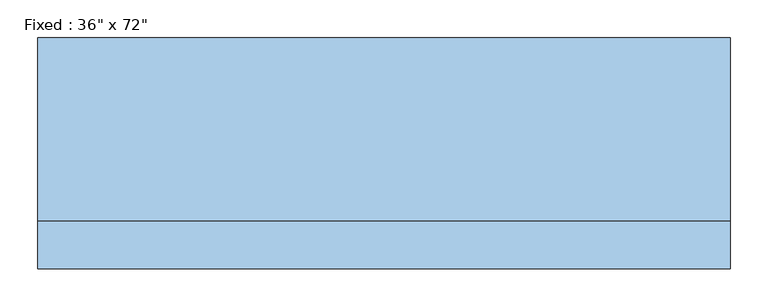
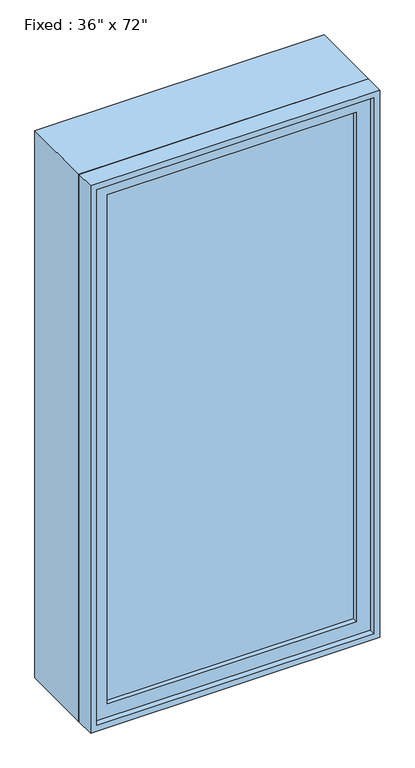
"""IFC4 building model written with IfcOpenShell, lengths in millimetres: window geometry."""

import ifcopenshell
import ifcopenshell.guid

model = None  # the IFC model being written
_history = None  # IfcOwnerHistory: only IFC2X3 demands one
_inside = {}  # id of a spatial element -> (the spatial element, [elements in it])
_under = {}  # id of a project, library or spatial element -> (it, [spatial elements below it])
_declared = {}  # id of a project -> (the project, [libraries it declares])
_typed = {}  # id of a type object -> (the type object, [elements of that type])
_made_of = {}  # id of a material, layer set ... -> (it, [elements and type objects made of it])


def new_model(schema):
    """Start an empty IFC model of exactly this schema.

    Asked for "IFC4X3", IfcOpenShell would pick the latest addendum, in which some entities
    have other attributes; the version numbers below select the first issue.
    IFC2X3 requires an IfcOwnerHistory on every rooted entity: one is made here for all.
    """
    global model, _history
    if schema == "IFC4X3":
        model = ifcopenshell.file(schema_version=(4, 3, 0, 0))
    else:
        model = ifcopenshell.file(schema=schema)
    _inside.clear()
    _under.clear()
    _declared.clear()
    _typed.clear()
    _made_of.clear()
    _history = None
    if model.schema == "IFC2X3":
        org = make("IfcOrganization", Name="unknown")
        user = make(
            "IfcPersonAndOrganization",
            ThePerson=make("IfcPerson", FamilyName="unknown"),
            TheOrganization=org,
        )
        app = make(
            "IfcApplication",
            ApplicationDeveloper=org,
            Version="unknown",
            ApplicationFullName="unknown",
            ApplicationIdentifier="unknown",
        )
        _history = make(
            "IfcOwnerHistory",
            OwningUser=user,
            OwningApplication=app,
            ChangeAction="ADDED",
            CreationDate=0,
        )
    return model


def make(cls, **values):
    """One entity of the class cls with the attributes given. An attribute that is None is left unset."""
    return model.create_entity(
        cls, **{name: value for name, value in values.items() if value is not None}
    )


def rooted(cls, **values):
    """An entity with a GlobalId (a new one), such as an element, a storey or a relation."""
    return make(cls, GlobalId=ifcopenshell.guid.new(), OwnerHistory=_history, **values)


def si_unit(unit_type, name, prefix=None):
    """IfcSIUnit, for example si_unit("LENGTHUNIT", "METRE", prefix="MILLI")."""
    return make("IfcSIUnit", UnitType=unit_type, Prefix=prefix, Name=name)


def assignment(units):
    """IfcUnitAssignment: the units of a project."""
    return None if units is None else make("IfcUnitAssignment", Units=units)


def point(xyz):
    """IfcCartesianPoint."""
    return None if xyz is None else make("IfcCartesianPoint", Coordinates=xyz)


def direction(xyz):
    """IfcDirection."""
    return None if xyz is None else make("IfcDirection", DirectionRatios=xyz)


def frame(location, z_axis=None, x_axis=None):
    """IfcAxis2Placement3D, a coordinate frame: its origin and axes. An axis left out is left unset."""
    return make(
        "IfcAxis2Placement3D",
        Location=point(location),
        Axis=direction(z_axis),
        RefDirection=direction(x_axis),
    )


def origin():
    """The frame at (0, 0, 0) with its axes left unset."""
    return frame((0.0, 0.0, 0.0))


def place(relative_to, where):
    """IfcLocalPlacement: puts the frame where relative to a parent placement (None: the world)."""
    return make(
        "IfcLocalPlacement", PlacementRelTo=relative_to, RelativePlacement=where
    )


def context(
    kind, dimensions, precision=None, world=None, true_north=None, identifier=None
):
    """IfcGeometricRepresentationContext, for example the 3D "Model" context."""
    return make(
        "IfcGeometricRepresentationContext",
        ContextIdentifier=identifier,
        ContextType=kind,
        CoordinateSpaceDimension=dimensions,
        Precision=precision,
        WorldCoordinateSystem=world,
        TrueNorth=true_north,
    )


def project(units=None, contexts=None):
    """IfcProject with its units and contexts."""
    return rooted(
        "IfcProject",
        Name="project",
        RepresentationContexts=contexts,
        UnitsInContext=assignment(units),
    )


def spatial(cls, under=None, at=None, **own):
    """A site, building, storey or space (cls), placed at a placement, below another one or the project."""
    s = rooted(cls, ObjectPlacement=at, **own)
    if under is not None:
        _under.setdefault(under.id(), (under, []))[1].append(s)
    return s


def polyline(points):
    """IfcPolyline through the points."""
    return make("IfcPolyline", Points=[point(p) for p in points])


def outline(outer, holes=None, kind="AREA"):
    """IfcArbitraryClosedProfileDef: a profile drawn as a closed curve; with holes, ...WithVoids."""
    if holes is None:
        return make("IfcArbitraryClosedProfileDef", ProfileType=kind, OuterCurve=outer)
    return make(
        "IfcArbitraryProfileDefWithVoids",
        ProfileType=kind,
        OuterCurve=outer,
        InnerCurves=holes,
    )


def extrude(swept, where, along, depth):
    """IfcExtrudedAreaSolid: the profile swept, set in the frame where, extruded along a direction by depth."""
    return make(
        "IfcExtrudedAreaSolid",
        SweptArea=swept,
        Position=where,
        ExtrudedDirection=direction(along),
        Depth=depth,
    )


def shape(context_of_items, identifier, shape_type, items):
    """IfcShapeRepresentation: the items that make up one representation, for example the "Body"."""
    return make(
        "IfcShapeRepresentation",
        ContextOfItems=context_of_items,
        RepresentationIdentifier=identifier,
        RepresentationType=shape_type,
        Items=items,
    )


def source(mapping_origin, context_of_items, identifier, shape_type, items):
    """IfcRepresentationMap: a shape defined once, which mapped items show again and again."""
    return make(
        "IfcRepresentationMap",
        MappingOrigin=mapping_origin,
        MappedRepresentation=shape(context_of_items, identifier, shape_type, items),
    )


def transform(
    local_origin,
    x_axis=None,
    y_axis=None,
    z_axis=None,
    scale=None,
    scale2=None,
    scale3=None,
    uniform=True,
):
    """IfcCartesianTransformationOperator3D, or its non-uniform kind. x_axis, y_axis, z_axis: its Axis1, 2, 3."""
    if uniform:
        return make(
            "IfcCartesianTransformationOperator3D",
            Axis1=direction(x_axis),
            Axis2=direction(y_axis),
            LocalOrigin=point(local_origin),
            Scale=scale,
            Axis3=direction(z_axis),
        )
    return make(
        "IfcCartesianTransformationOperator3DnonUniform",
        Axis1=direction(x_axis),
        Axis2=direction(y_axis),
        LocalOrigin=point(local_origin),
        Scale=scale,
        Axis3=direction(z_axis),
        Scale2=scale2,
        Scale3=scale3,
    )


def mapped(mapping_source, mapping_target):
    """IfcMappedItem: shows the shape of a source again, moved by a transform."""
    return make(
        "IfcMappedItem", MappingSource=mapping_source, MappingTarget=mapping_target
    )


def made_of(thing, what):
    """Note that an element or type object is made of a material, layer set ...; save() writes the relation."""
    if what is not None:
        _made_of.setdefault(what.id(), (what, []))[1].append(thing)
    return thing


def element(
    cls,
    number,
    at=None,
    inside=None,
    cuts=None,
    type_object=None,
    material=None,
    context=None,
    identifier="Body",
    shape_type=None,
    held_by="IfcProductDefinitionShape",
    body=None,
    shapes=None,
    **own,
):
    """One element of the class cls, such as IfcWall. Its Tag is "e" and its number.

    at: its placement. inside: the storey or other place that contains it. cuts: it is an
    opening in that element (IfcRelVoidsElement). A single representation is given by context,
    identifier, shape_type and body (its items); several are given by shapes. held_by: the class
    of the entity that holds the representations. save() writes the other relations.
    """
    e = rooted(cls, Tag="e%d" % number, ObjectPlacement=at, **own)
    if body is not None:
        shapes = [shape(context, identifier, shape_type, body)]
    if shapes is not None:
        e.Representation = make(held_by, Representations=shapes)
    if inside is not None:
        _inside.setdefault(inside.id(), (inside, []))[1].append(e)
    if cuts is not None:
        rooted(
            "IfcRelVoidsElement", RelatingBuildingElement=cuts, RelatedOpeningElement=e
        )
    if type_object is not None:
        _typed.setdefault(type_object.id(), (type_object, []))[1].append(e)
    return made_of(e, material)


def aggregate(whole, parts):
    """IfcRelAggregates: a whole, such as a stair, and the parts it consists of."""
    return rooted("IfcRelAggregates", RelatingObject=whole, RelatedObjects=parts)


def save(model, path):
    """Write the relations noted so far, then the file.

    IfcRelAggregates (storeys below a building ...), IfcRelContainedInSpatialStructure (elements
    in a storey), IfcRelDefinesByType, IfcRelAssociatesMaterial and IfcRelDeclares: one each for
    every whole, place, type object, material and project.
    """
    for whole, parts in _under.values():
        aggregate(whole, parts)
    for where, things in _inside.values():
        rooted(
            "IfcRelContainedInSpatialStructure",
            RelatedElements=things,
            RelatingStructure=where,
        )
    for kind, things in _typed.values():
        rooted("IfcRelDefinesByType", RelatedObjects=things, RelatingType=kind)
    for what, things in _made_of.values():
        rooted("IfcRelAssociatesMaterial", RelatedObjects=things, RelatingMaterial=what)
    for by, libraries in _declared.values():
        rooted("IfcRelDeclares", RelatingContext=by, RelatedDefinitions=libraries)
    model.write(path)


def window_9a1f8bc2(model_context):
    return source(origin(), model_context, "Body", "SweptSolid", [
        extrude(outline(polyline([(355.6, -104.775), (355.6, -117.475), (-431.8, -117.475), (-431.8, -104.775), (355.6, -104.775)])), frame((0.0, 0.0, 368.3), z_axis=(0.0, 0.0, 1.0), x_axis=(1.0, 0.0, 0.0)), (0.0, 0.0, 1.0), 1701.8),
        extrude(outline(polyline([(2114.55, -476.25), (323.85, -476.25), (323.85, 400.05), (2114.55, 400.05), (2114.55, -476.25)]), holes=[polyline([(2070.1, -431.8), (2070.1, 355.6), (368.3, 355.6), (368.3, -431.8), (2070.1, -431.8)])]), frame((0.0, -133.35, 0.0), z_axis=(0.0, 1.0, 0.0), x_axis=(0.0, 0.0, 1.0)), (0.0, 0.0, 1.0), 44.45),
        extrude(outline(polyline([(2133.6, -495.3), (304.8, -495.3), (304.8, 419.1), (2133.6, 419.1), (2133.6, -495.3)]), holes=[polyline([(2101.85, -463.55), (2101.85, 387.35), (336.55, 387.35), (336.55, -463.55), (2101.85, -463.55)])]), frame((0.0, -88.9, 0.0), z_axis=(0.0, 1.0, 0.0), x_axis=(0.0, 0.0, 1.0)), (0.0, 0.0, 1.0), 241.3),
        extrude(outline(polyline([(2133.6, 419.1), (2133.6, -495.3), (304.8, -495.3), (304.8, 419.1), (2133.6, 419.1)]), holes=[polyline([(2114.55, 400.05), (323.85, 400.05), (323.85, -476.25), (2114.55, -476.25), (2114.55, 400.05)])]), frame((0.0, -152.4, 0.0), z_axis=(0.0, 1.0, 0.0), x_axis=(0.0, 0.0, 1.0)), (0.0, 0.0, 1.0), 63.5),
    ])


if __name__ == "__main__":
    model = new_model("IFC4")
    model_context = context("Model", 3, world=origin())
    ifc_project = project(units=[si_unit("LENGTHUNIT", "METRE", prefix="MILLI")], contexts=[model_context])
    site = spatial("IfcSite", under=ifc_project)
    building = spatial("IfcBuilding", under=site)
    placement = place(None, origin())
    window_shape = window_9a1f8bc2(model_context)
    element("IfcWindow", 1, ObjectType="Fixed : 36\" x 72\"", at=placement, inside=building, context=model_context, shape_type="MappedRepresentation", body=[
        mapped(window_shape, transform((0.0, 0.0, 0.0), x_axis=(1.0, 0.0, 0.0), y_axis=(0.0, 1.0, 0.0), z_axis=(0.0, 0.0, 1.0))),
    ])
    save(model, "model.ifc")

# Revit data of these elements
# Type "Fixed : 36\" x 72\""
#   Type Mark = "18"
#   Construction Type Id = "GSP4R"
#   Assembly Code = "B2020100"
#   Analytic Construction = "1/8 in Pilkington single glazing"
#   Visual Light Transmittance = 0.9
#   Solar Heat Gain Coefficient = 0.78
#   Heat Transfer Coefficient (U) = 0.6496 BTU/(h·ft²·°F)
#   Height = 6' - 0"
#   Default Sill Height = 1' - 0"
#   Width = 3' - 0"
#   Window Inset = 0' - 0 3/4"
#   Define Thermal Properties by = 1
#   Define Thermal Properties by = 1
#   Glass Pane Material = Glass
#   Sash Material = Sash
#   Wall Closure = (empty or 0)
# Element 1 (IfcWindow, "Fixed : 36\" x 72\"")
#   Materials on its faces: "Sash", "Glass"
# Materials
#   "Glass": class "Glass", colour RGB 0 0 255, transparency 0.75, Description = "Soda Lime Glass", Cost = 0
#   "Sash": class "Wood", colour RGB 224 178 126, transparency 0, Cost = 0
